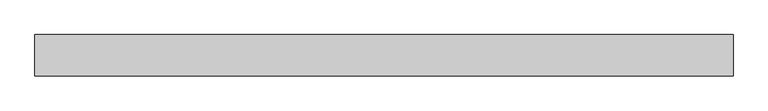
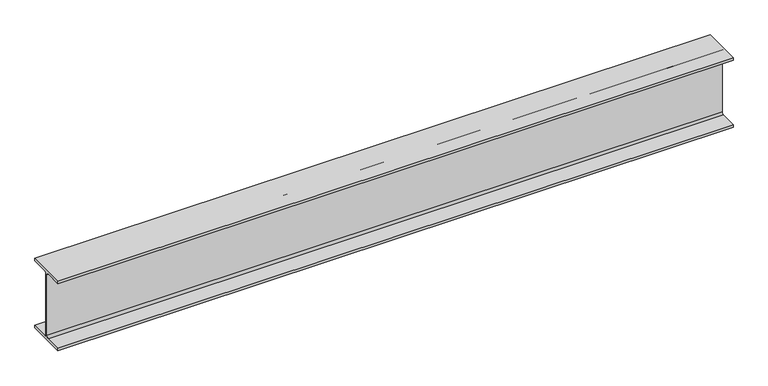
"""IFC4 building model written with IfcOpenShell, lengths in millimetres: beam geometry, Steel Beam_H-KSD3502 : H_SB_ASB_H-250x125x6x9."""

from ifc_helpers import new_model, si_unit, point, frame, frame_2d, origin, place, context, project, spatial, polyline, circle_curve, trimmed, segment, composite_curve, outline, extrude, source, transform, mapped, element, save


def beam_b824a9ea(model_context):
    return source(origin(), model_context, "Body", "SweptSolid", [
        extrude(outline(composite_curve([segment(polyline([(82.5, -141.5), (82.5, -151.7), (-82.5, -151.7), (-82.5, -141.5), (-11.9, -141.5)]), True, "CONTINUOUS"), segment(trimmed(circle_curve(frame_2d((-11.9, -132.6)), 8.9), [point((-11.9, -141.5))], [point((-3.0, -132.6))], True, "CARTESIAN"), True, "CONTINUOUS"), segment(polyline([(-3.0, -132.6), (-3.0, 132.6)]), True, "CONTINUOUS"), segment(trimmed(circle_curve(frame_2d((-11.9, 132.6)), 8.9), [point((-3.0, 132.6))], [point((-11.9, 141.5))], True, "CARTESIAN"), True, "CONTINUOUS"), segment(polyline([(-11.9, 141.5), (-82.5, 141.5), (-82.5, 151.7), (82.5, 151.7), (82.5, 141.5), (11.9, 141.5)]), True, "CONTINUOUS"), segment(trimmed(circle_curve(frame_2d((11.9, 132.6)), 8.9), [point((11.9, 141.5))], [point((3.0, 132.6))], True, "CARTESIAN"), True, "CONTINUOUS"), segment(polyline([(3.0, 132.6), (3.0, -132.6)]), True, "CONTINUOUS"), segment(trimmed(circle_curve(frame_2d((11.9, -132.6)), 8.9), [point((3.0, -132.6))], [point((11.9, -141.5))], True, "CARTESIAN"), True, "CONTINUOUS"), segment(polyline([(11.9, -141.5), (82.5, -141.5)]), True, "CONTINUOUS")], self_intersect=False)), frame((-1382.2982577, 0.0, 0.0), z_axis=(1.0, 0.0, 0.0), x_axis=(0.0, 1.0, 0.0)), (0.0, 0.0, 1.0), 2794.5982507),
    ])


if __name__ == "__main__":
    model = new_model("IFC4")
    model_context = context("Model", 3, world=origin())
    ifc_project = project(units=[si_unit("LENGTHUNIT", "METRE", prefix="MILLI")], contexts=[model_context])
    site = spatial("IfcSite", under=ifc_project)
    building = spatial("IfcBuilding", under=site)
    placement = place(None, origin())
    beam_shape = beam_b824a9ea(model_context)
    element("IfcBeam", 1, ObjectType="Steel Beam_H-KSD3502 : H_SB_ASB_H-250x125x6x9", at=placement, inside=building, context=model_context, shape_type="MappedRepresentation", body=[
        mapped(beam_shape, transform((0.0, 0.0, 0.0), x_axis=(1.0, 0.0, 0.0), y_axis=(0.0, 1.0, 0.0), z_axis=(0.0, 0.0, 1.0))),
    ])
    save(model, "model.ifc")

# Revit data of these elements
# Type "Steel Beam_H-KSD3502 : H_SB_ASB_H-250x125x6x9"
#   Width = 12.5 cm
#   Web Thickness = 0.6 cm
#   Web Fillet = 1.2 cm
#   Warping Constant = 42539.8 cm⁶
#   Torsional Moment of Inertia = 7.8102 cm⁴
#   Torsional Modulus = 1.0 cm³
#   Section Area = 37.66 cm²
#   Plastic Modulus weak axis = 73.1 cm³
#   Plastic Modulus strong axis = 366.0 cm³
#   Perimeter = 0.97 m²/m
#   Nominal Weight = 29.60 kgf/m
#   Moment of Inertia weak axis = 294.00 cm⁴
#   Moment of Inertia strong axis = 4050.00 cm⁴
#   Height = 25.0 cm
#   Flange Thickness = 0.9 cm
#   Elastic Modulus weak axis = 47.0 cm³
#   Elastic Modulus strong axis = 324.0 cm³
#   Centroid Vertical = 12.5 cm
#   Centroid Horizontal = 6.25 cm
#   Length [instance default] = 1.5240 m
#   Structural Material [instance default] = Steel, 45-345
#   Assembly Code = ""
# Element 1 (IfcBeam, "Steel Beam_H-KSD3502 : H_SB_ASB_H-250x125x6x9")
#   Structural Material = none
# Materials
#   "Steel, 45-345": class "Metal", colour RGB 189 187 185, transparency 0, Description = "Steel 345 MPa", Cost = 0
